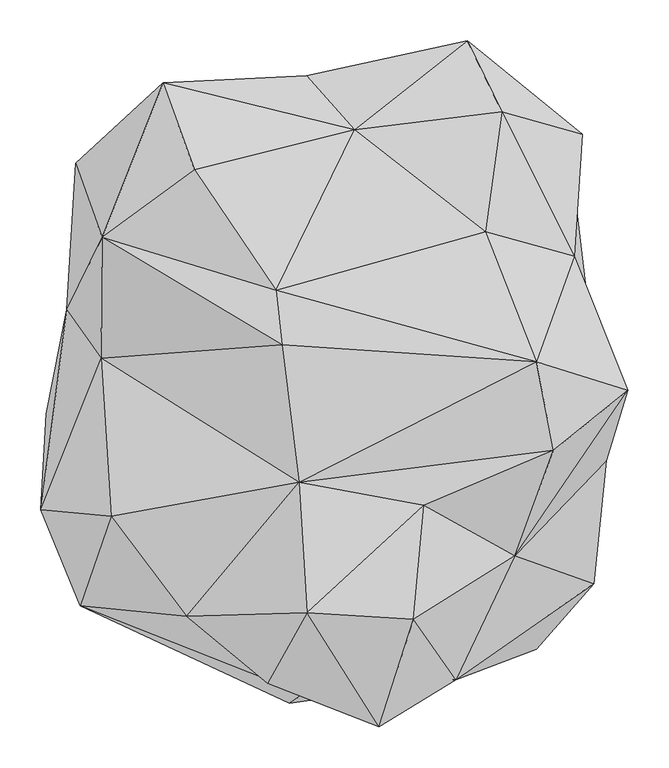
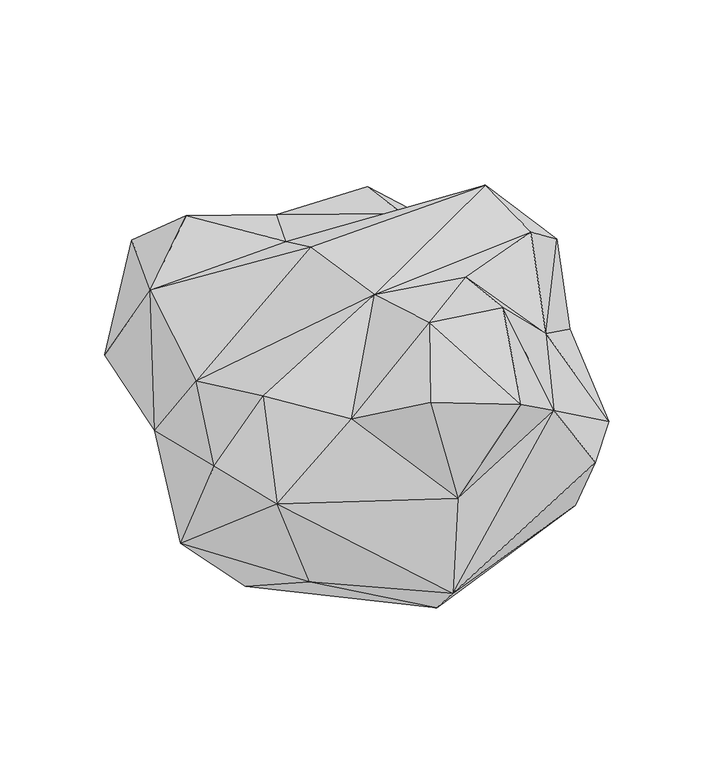
"""IFC4 building model written with IfcOpenShell, lengths in millimetres: geographic element geometry, Enscape AssetDefinition - Asparagaceae 001 Agave : Enscape AssetDefinition - Asparagaceae 001 Agave."""

from ifc_helpers import new_model, si_unit, origin, place, context, project, spatial, faceted_brep, source, transform, mapped, element, save


def geographic_element_a6fbcd7a(model_context):
    return source(origin(), model_context, "Body", "Brep", [
        faceted_brep([(-83.9166865, 203.263849, 0.0), (12.647056, 313.811481, 48.0152518), (67.6679313, 62.6604483, 0.0), (180.0118238, 64.2274469, 0.0), (-240.9703434, 321.6060698, 224.4298905), (218.8661695, 340.318799, 147.609368), (130.1935166, 418.3222353, 188.9963597), (54.3873757, -37.3966545, 0.0), (-309.7500205, 30.4520428, 66.9589713), (-282.8032076, -74.3769556, 51.3344258), (-68.5941651, -314.8398399, 80.1332444), (281.7476392, -32.8720361, 60.0785054), (227.4366021, -243.2648838, 132.4731708), (-372.3214567, -22.7501001, 135.3752464), (-245.0786829, -213.5978639, 130.9934407), (-74.6905804, -376.1395216, 147.9662508), (297.0918119, -230.159983, 264.4174993), (226.5083939, -310.1032972, 257.6498091), (-58.5948005, -364.6009266, 320.3084469), (-330.3538561, -257.1682334, 339.8004174), (128.2582879, -347.3773599, 415.8658981), (-292.5794125, -147.57514, 469.5923924), (-378.6310256, -139.8030221, 359.0724468), (-200.5006969, -269.4469392, 466.7710066), (-101.5319452, -351.2604833, 514.261961), (34.3744606, -404.9287438, 495.1784015), (-53.6577664, -265.4434741, 601.4473438), (-63.4572953, -105.9724018, 562.3546839), (-305.0922155, 45.468282, 386.8079782), (-347.0320106, 104.5354754, 268.994689), (-303.935796, 193.1274682, 474.0562737), (-84.1022134, 61.705336, 560.44662), (-336.4052773, 283.3358645, 304.1164875), (-91.2186354, 128.3842325, 533.411622), (-190.626651, 275.4265964, 529.8674107), (-229.4352949, 381.8665445, 430.6333363), (226.3577729, 40.6467356, 585.7200027), (164.413169, 199.5292455, 455.4721117), (4.5721261, 324.2405057, 433.6276054), (-53.8770929, 389.9331093, 315.5574501), (-227.6405096, 376.0583401, 284.8320007), (142.7014321, 432.5819612, 292.3455834), (184.7079694, 346.2255597, 411.3186896), (272.7532089, 169.5409268, 383.0037415), (283.0359936, 318.8481033, 317.0358241), (273.9757001, 240.0513738, 187.9213154), (338.1246328, 6.1014961, 462.3352885), (312.279731, -80.1761523, 348.0335176), (200.6652653, -196.0080713, 448.3486712), (247.2611368, -67.0667812, 551.8904924), (89.1786218, -134.4338804, 560.2785349), (76.2959495, -273.5785842, 589.6103978)], [[[0, 1, 2]], [[2, 1, 3]], [[4, 1, 0]], [[1, 5, 3]], [[1, 6, 5]], [[1, 4, 6]], [[7, 0, 2]], [[7, 2, 3]], [[4, 0, 8]], [[8, 0, 7]], [[9, 7, 10]], [[7, 11, 12]], [[11, 7, 3]], [[9, 8, 7]], [[12, 10, 7]], [[8, 13, 4]], [[13, 8, 9]], [[9, 14, 13]], [[14, 9, 10]], [[10, 12, 15]], [[10, 15, 14]], [[11, 16, 12]], [[12, 17, 15]], [[17, 12, 16]], [[15, 18, 19]], [[14, 15, 19]], [[17, 20, 15]], [[18, 15, 20]], [[13, 14, 19]], [[21, 22, 19]], [[22, 13, 19]], [[18, 23, 19]], [[21, 19, 23]], [[18, 24, 23]], [[18, 25, 24]], [[18, 20, 25]], [[23, 24, 26]], [[23, 26, 27]], [[21, 23, 27]], [[21, 28, 22]], [[21, 27, 28]], [[28, 29, 22]], [[13, 22, 29]], [[28, 30, 29]], [[30, 28, 31]], [[27, 31, 28]], [[4, 29, 32]], [[29, 4, 13]], [[29, 30, 32]], [[30, 33, 34]], [[35, 30, 34]], [[30, 31, 33]], [[32, 30, 35]], [[31, 36, 33]], [[27, 36, 31]], [[37, 38, 33]], [[33, 36, 37]], [[34, 33, 38]], [[34, 38, 35]], [[39, 35, 38]], [[32, 35, 40]], [[40, 35, 39]], [[4, 32, 40]], [[4, 40, 39]], [[4, 39, 6]], [[39, 41, 6]], [[39, 38, 41]], [[38, 42, 41]], [[38, 37, 42]], [[37, 36, 43]], [[43, 42, 37]], [[41, 42, 44]], [[43, 44, 42]], [[6, 41, 5]], [[5, 41, 44]], [[44, 45, 5]], [[45, 44, 43]], [[46, 47, 43]], [[43, 36, 46]], [[47, 45, 43]], [[5, 45, 3]], [[11, 3, 45]], [[11, 45, 47]], [[47, 46, 48]], [[48, 16, 47]], [[16, 11, 47]], [[48, 46, 49]], [[46, 36, 49]], [[27, 49, 36]], [[49, 50, 48]], [[50, 49, 27]], [[48, 51, 20]], [[51, 48, 50]], [[20, 16, 48]], [[20, 17, 16]], [[20, 51, 25]], [[50, 26, 51]], [[26, 25, 51]], [[26, 50, 27]], [[24, 25, 26]]]),
    ])


if __name__ == "__main__":
    model = new_model("IFC4")
    model_context = context("Model", 3, world=origin())
    ifc_project = project(units=[si_unit("LENGTHUNIT", "METRE", prefix="MILLI")], contexts=[model_context])
    site = spatial("IfcSite", under=ifc_project)
    building = spatial("IfcBuilding", under=site)
    placement = place(None, origin())
    geographic_element_shape = geographic_element_a6fbcd7a(model_context)
    element("IfcGeographicElement", 1, ObjectType="Enscape AssetDefinition - Asparagaceae 001 Agave : Enscape AssetDefinition - Asparagaceae 001 Agave", at=placement, inside=building, context=model_context, shape_type="MappedRepresentation", body=[
        mapped(geographic_element_shape, transform((0.0, 0.0, 0.0), x_axis=(1.0, 0.0, 0.0), y_axis=(0.0, 1.0, 0.0), z_axis=(0.0, 0.0, 1.0))),
    ])
    save(model, "model.ifc")

# Revit data of these elements
# Type "Enscape AssetDefinition - Asparagaceae 001 Agave : Enscape AssetDefinition - Asparagaceae 001 Agave"
#   EnscapeAssetSource = "REMOTE"
#   EnscapeAssetId = "6d861ce6-d1f1-4992-8acd-35a045128a82"
#   Height = 0.601447 m
#   EnscapeNativeAssetHeight = 0.601447 m
#   Default Elevation = 0
